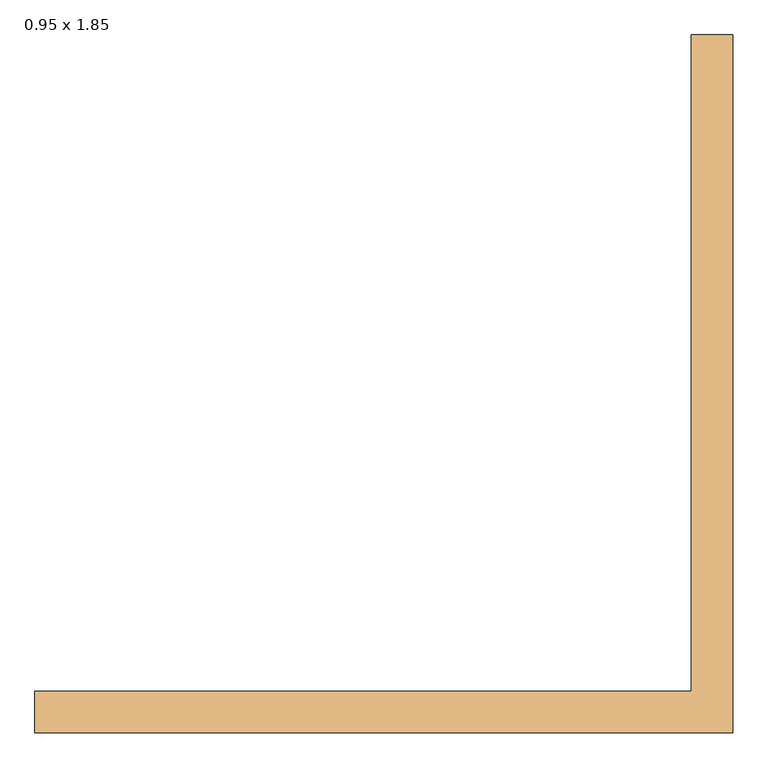
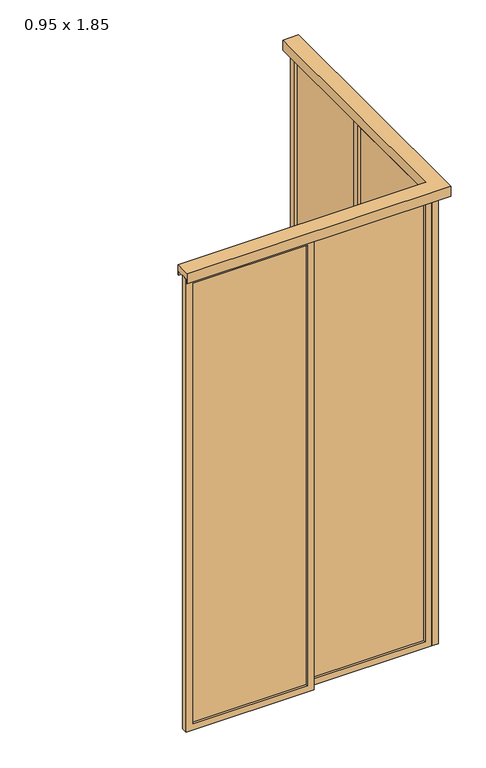
"""IFC4 building model written with IfcOpenShell, lengths in millimetres: door geometry, CC_ND-200_BOX-L-BANHEIRO : 0.95 x 1.85."""

import ifcopenshell
import ifcopenshell.guid

model = None  # the IFC model being written
_history = None  # IfcOwnerHistory: only IFC2X3 demands one
_inside = {}  # id of a spatial element -> (the spatial element, [elements in it])
_under = {}  # id of a project, library or spatial element -> (it, [spatial elements below it])
_declared = {}  # id of a project -> (the project, [libraries it declares])
_typed = {}  # id of a type object -> (the type object, [elements of that type])
_made_of = {}  # id of a material, layer set ... -> (it, [elements and type objects made of it])


def new_model(schema):
    """Start an empty IFC model of exactly this schema.

    Asked for "IFC4X3", IfcOpenShell would pick the latest addendum, in which some entities
    have other attributes; the version numbers below select the first issue.
    IFC2X3 requires an IfcOwnerHistory on every rooted entity: one is made here for all.
    """
    global model, _history
    if schema == "IFC4X3":
        model = ifcopenshell.file(schema_version=(4, 3, 0, 0))
    else:
        model = ifcopenshell.file(schema=schema)
    _inside.clear()
    _under.clear()
    _declared.clear()
    _typed.clear()
    _made_of.clear()
    _history = None
    if model.schema == "IFC2X3":
        org = make("IfcOrganization", Name="unknown")
        user = make(
            "IfcPersonAndOrganization",
            ThePerson=make("IfcPerson", FamilyName="unknown"),
            TheOrganization=org,
        )
        app = make(
            "IfcApplication",
            ApplicationDeveloper=org,
            Version="unknown",
            ApplicationFullName="unknown",
            ApplicationIdentifier="unknown",
        )
        _history = make(
            "IfcOwnerHistory",
            OwningUser=user,
            OwningApplication=app,
            ChangeAction="ADDED",
            CreationDate=0,
        )
    return model


def make(cls, **values):
    """One entity of the class cls with the attributes given. An attribute that is None is left unset."""
    return model.create_entity(
        cls, **{name: value for name, value in values.items() if value is not None}
    )


def rooted(cls, **values):
    """An entity with a GlobalId (a new one), such as an element, a storey or a relation."""
    return make(cls, GlobalId=ifcopenshell.guid.new(), OwnerHistory=_history, **values)


def si_unit(unit_type, name, prefix=None):
    """IfcSIUnit, for example si_unit("LENGTHUNIT", "METRE", prefix="MILLI")."""
    return make("IfcSIUnit", UnitType=unit_type, Prefix=prefix, Name=name)


def assignment(units):
    """IfcUnitAssignment: the units of a project."""
    return None if units is None else make("IfcUnitAssignment", Units=units)


def point(xyz):
    """IfcCartesianPoint."""
    return None if xyz is None else make("IfcCartesianPoint", Coordinates=xyz)


def direction(xyz):
    """IfcDirection."""
    return None if xyz is None else make("IfcDirection", DirectionRatios=xyz)


def frame(location, z_axis=None, x_axis=None):
    """IfcAxis2Placement3D, a coordinate frame: its origin and axes. An axis left out is left unset."""
    return make(
        "IfcAxis2Placement3D",
        Location=point(location),
        Axis=direction(z_axis),
        RefDirection=direction(x_axis),
    )


def origin():
    """The frame at (0, 0, 0) with its axes left unset."""
    return frame((0.0, 0.0, 0.0))


def origin_with_axes():
    """The frame at (0, 0, 0) with the z axis (0, 0, 1) and the x axis (1, 0, 0) written out."""
    return frame((0.0, 0.0, 0.0), z_axis=(0.0, 0.0, 1.0), x_axis=(1.0, 0.0, 0.0))


def place(relative_to, where):
    """IfcLocalPlacement: puts the frame where relative to a parent placement (None: the world)."""
    return make(
        "IfcLocalPlacement", PlacementRelTo=relative_to, RelativePlacement=where
    )


def context(
    kind, dimensions, precision=None, world=None, true_north=None, identifier=None
):
    """IfcGeometricRepresentationContext, for example the 3D "Model" context."""
    return make(
        "IfcGeometricRepresentationContext",
        ContextIdentifier=identifier,
        ContextType=kind,
        CoordinateSpaceDimension=dimensions,
        Precision=precision,
        WorldCoordinateSystem=world,
        TrueNorth=true_north,
    )


def project(units=None, contexts=None):
    """IfcProject with its units and contexts."""
    return rooted(
        "IfcProject",
        Name="project",
        RepresentationContexts=contexts,
        UnitsInContext=assignment(units),
    )


def spatial(cls, under=None, at=None, **own):
    """A site, building, storey or space (cls), placed at a placement, below another one or the project."""
    s = rooted(cls, ObjectPlacement=at, **own)
    if under is not None:
        _under.setdefault(under.id(), (under, []))[1].append(s)
    return s


def polyline(points):
    """IfcPolyline through the points."""
    return make("IfcPolyline", Points=[point(p) for p in points])


def outline(outer, holes=None, kind="AREA"):
    """IfcArbitraryClosedProfileDef: a profile drawn as a closed curve; with holes, ...WithVoids."""
    if holes is None:
        return make("IfcArbitraryClosedProfileDef", ProfileType=kind, OuterCurve=outer)
    return make(
        "IfcArbitraryProfileDefWithVoids",
        ProfileType=kind,
        OuterCurve=outer,
        InnerCurves=holes,
    )


def extrude(swept, where, along, depth):
    """IfcExtrudedAreaSolid: the profile swept, set in the frame where, extruded along a direction by depth."""
    return make(
        "IfcExtrudedAreaSolid",
        SweptArea=swept,
        Position=where,
        ExtrudedDirection=direction(along),
        Depth=depth,
    )


def faces_of(points, faces, orient=None, outer=None):
    """IfcFace entities. A face is a list of loops; a loop is a list of indices into points, from 0.

    orient and outer hold one flag for each loop. By default every Orientation is true, the
    first loop of a face is its IfcFaceOuterBound and the others are IfcFaceBound.
    """
    made = []
    for i, loops in enumerate(faces):
        bounds = []
        for j, loop in enumerate(loops):
            is_outer = j == 0 if outer is None else outer[i][j]
            bounds.append(
                make(
                    "IfcFaceOuterBound" if is_outer else "IfcFaceBound",
                    Bound=make("IfcPolyLoop", Polygon=[points[k] for k in loop]),
                    Orientation=True if orient is None else orient[i][j],
                )
            )
        made.append(make("IfcFace", Bounds=bounds))
    return made


def faceted_brep(points, faces, orient=None, outer=None, voids=None):
    """IfcFacetedBrep: a solid bounded by flat faces; with voids (closed shells), ...WithVoids."""
    shared = [point(p) for p in points]
    hull = make("IfcClosedShell", CfsFaces=faces_of(shared, faces, orient, outer))
    if voids is None:
        return make("IfcFacetedBrep", Outer=hull)
    return make(
        "IfcFacetedBrepWithVoids",
        Outer=hull,
        Voids=[
            make(cls, CfsFaces=faces_of(shared, fs, o, b)) for cls, fs, o, b in voids
        ],
    )


def shape(context_of_items, identifier, shape_type, items):
    """IfcShapeRepresentation: the items that make up one representation, for example the "Body"."""
    return make(
        "IfcShapeRepresentation",
        ContextOfItems=context_of_items,
        RepresentationIdentifier=identifier,
        RepresentationType=shape_type,
        Items=items,
    )


def source(mapping_origin, context_of_items, identifier, shape_type, items):
    """IfcRepresentationMap: a shape defined once, which mapped items show again and again."""
    return make(
        "IfcRepresentationMap",
        MappingOrigin=mapping_origin,
        MappedRepresentation=shape(context_of_items, identifier, shape_type, items),
    )


def transform(
    local_origin,
    x_axis=None,
    y_axis=None,
    z_axis=None,
    scale=None,
    scale2=None,
    scale3=None,
    uniform=True,
):
    """IfcCartesianTransformationOperator3D, or its non-uniform kind. x_axis, y_axis, z_axis: its Axis1, 2, 3."""
    if uniform:
        return make(
            "IfcCartesianTransformationOperator3D",
            Axis1=direction(x_axis),
            Axis2=direction(y_axis),
            LocalOrigin=point(local_origin),
            Scale=scale,
            Axis3=direction(z_axis),
        )
    return make(
        "IfcCartesianTransformationOperator3DnonUniform",
        Axis1=direction(x_axis),
        Axis2=direction(y_axis),
        LocalOrigin=point(local_origin),
        Scale=scale,
        Axis3=direction(z_axis),
        Scale2=scale2,
        Scale3=scale3,
    )


def mapped(mapping_source, mapping_target):
    """IfcMappedItem: shows the shape of a source again, moved by a transform."""
    return make(
        "IfcMappedItem", MappingSource=mapping_source, MappingTarget=mapping_target
    )


def made_of(thing, what):
    """Note that an element or type object is made of a material, layer set ...; save() writes the relation."""
    if what is not None:
        _made_of.setdefault(what.id(), (what, []))[1].append(thing)
    return thing


def element(
    cls,
    number,
    at=None,
    inside=None,
    cuts=None,
    type_object=None,
    material=None,
    context=None,
    identifier="Body",
    shape_type=None,
    held_by="IfcProductDefinitionShape",
    body=None,
    shapes=None,
    **own,
):
    """One element of the class cls, such as IfcWall. Its Tag is "e" and its number.

    at: its placement. inside: the storey or other place that contains it. cuts: it is an
    opening in that element (IfcRelVoidsElement). A single representation is given by context,
    identifier, shape_type and body (its items); several are given by shapes. held_by: the class
    of the entity that holds the representations. save() writes the other relations.
    """
    e = rooted(cls, Tag="e%d" % number, ObjectPlacement=at, **own)
    if body is not None:
        shapes = [shape(context, identifier, shape_type, body)]
    if shapes is not None:
        e.Representation = make(held_by, Representations=shapes)
    if inside is not None:
        _inside.setdefault(inside.id(), (inside, []))[1].append(e)
    if cuts is not None:
        rooted(
            "IfcRelVoidsElement", RelatingBuildingElement=cuts, RelatedOpeningElement=e
        )
    if type_object is not None:
        _typed.setdefault(type_object.id(), (type_object, []))[1].append(e)
    return made_of(e, material)


def aggregate(whole, parts):
    """IfcRelAggregates: a whole, such as a stair, and the parts it consists of."""
    return rooted("IfcRelAggregates", RelatingObject=whole, RelatedObjects=parts)


def save(model, path):
    """Write the relations noted so far, then the file.

    IfcRelAggregates (storeys below a building ...), IfcRelContainedInSpatialStructure (elements
    in a storey), IfcRelDefinesByType, IfcRelAssociatesMaterial and IfcRelDeclares: one each for
    every whole, place, type object, material and project.
    """
    for whole, parts in _under.values():
        aggregate(whole, parts)
    for where, things in _inside.values():
        rooted(
            "IfcRelContainedInSpatialStructure",
            RelatedElements=things,
            RelatingStructure=where,
        )
    for kind, things in _typed.values():
        rooted("IfcRelDefinesByType", RelatedObjects=things, RelatingType=kind)
    for what, things in _made_of.values():
        rooted("IfcRelAssociatesMaterial", RelatedObjects=things, RelatingMaterial=what)
    for by, libraries in _declared.values():
        rooted("IfcRelDeclares", RelatingContext=by, RelatedDefinitions=libraries)
    model.write(path)


def door_0_95_x_1_85_64086e03(model_context):
    return source(origin(), model_context, "Body", "SolidModel", [
        extrude(outline(polyline([(975.0, 50.0), (975.0, 25.0), (950.0, 25.0), (950.0, 50.0), (975.0, 50.0)])), origin_with_axes(), (0.0, 0.0, 1.0), 1825.0),
        extrude(outline(polyline([(965.0, 527.5), (965.0, 60.0), (960.0, 60.0), (960.0, 527.5), (965.0, 527.5)])), frame((0.0, 0.0, 10.0), z_axis=(0.0, 0.0, 1.0), x_axis=(1.0, 0.0, 0.0)), (0.0, 0.0, 1.0), 1805.0),
        faceted_brep([(975.0, 512.5, 1800.0), (965.0, 512.5, 1800.0), (965.0, 512.5, 25.0), (975.0, 512.5, 25.0), (965.0, 527.5, 1815.0), (965.0, 527.5, 10.0), (965.0, 60.0, 10.0), (965.0, 60.0, 1815.0), (965.0, 75.0, 1800.0), (965.0, 75.0, 25.0), (975.0, 75.0, 25.0), (975.0, 50.0, 1825.0), (975.0, 50.0, 0.0), (975.0, 537.5, 0.0), (975.0, 537.5, 1825.0), (975.0, 75.0, 1800.0), (950.0, 537.5, 1825.0), (950.0, 537.5, 0.0), (950.0, 50.0, 0.0), (950.0, 50.0, 1825.0), (950.0, 75.0, 1800.0), (950.0, 75.0, 25.0), (950.0, 512.5, 25.0), (950.0, 512.5, 1800.0), (960.0, 75.0, 25.0), (960.0, 75.0, 1800.0), (960.0, 512.5, 25.0), (960.0, 512.5, 1800.0), (960.0, 527.5, 1815.0), (960.0, 527.5, 10.0), (960.0, 60.0, 1815.0), (960.0, 60.0, 10.0)], [[[0, 1, 2, 3]], [[4, 5, 6, 7], [8, 9, 2, 1]], [[3, 2, 9, 10]], [[11, 12, 13, 14], [0, 3, 10, 15]], [[16, 14, 13, 17]], [[17, 13, 12, 18]], [[16, 17, 18, 19], [20, 21, 22, 23]], [[10, 9, 8, 15]], [[18, 12, 11, 19]], [[24, 21, 20, 25]], [[26, 22, 21, 24]], [[27, 23, 22, 26]], [[4, 28, 29, 5]], [[30, 31, 29, 28], [27, 26, 24, 25]], [[5, 29, 31, 6]], [[6, 31, 30, 7]], [[15, 8, 1, 0]], [[19, 11, 14, 16]], [[7, 30, 28, 4]], [[25, 20, 23, 27]]]),
        extrude(outline(polyline([(990.0, 990.0), (990.0, 522.5), (985.0, 522.5), (985.0, 990.0), (990.0, 990.0)])), frame((0.0, 0.0, 10.0), z_axis=(0.0, 0.0, 1.0), x_axis=(1.0, 0.0, 0.0)), (0.0, 0.0, 1.0), 1805.0),
        faceted_brep([(1000.0, 975.0, 1800.0), (990.0, 975.0, 1800.0), (990.0, 975.0, 25.0), (1000.0, 975.0, 25.0), (990.0, 990.0, 1815.0), (990.0, 990.0, 10.0), (990.0, 522.5, 10.0), (990.0, 522.5, 1815.0), (990.0, 537.5, 1800.0), (990.0, 537.5, 25.0), (1000.0, 537.5, 25.0), (1000.0, 512.5, 1825.0), (1000.0, 512.5, 0.0), (1000.0, 1000.0, 0.0), (1000.0, 1000.0, 1825.0), (1000.0, 537.5, 1800.0), (975.0, 1000.0, 1825.0), (975.0, 1000.0, 0.0), (975.0, 512.5, 0.0), (975.0, 512.5, 1825.0), (975.0, 537.5, 1800.0), (975.0, 537.5, 25.0), (975.0, 975.0, 25.0), (975.0, 975.0, 1800.0), (985.0, 537.5, 25.0), (985.0, 537.5, 1800.0), (985.0, 975.0, 25.0), (985.0, 975.0, 1800.0), (985.0, 990.0, 1815.0), (985.0, 990.0, 10.0), (985.0, 522.5, 1815.0), (985.0, 522.5, 10.0)], [[[0, 1, 2, 3]], [[4, 5, 6, 7], [8, 9, 2, 1]], [[3, 2, 9, 10]], [[11, 12, 13, 14], [0, 3, 10, 15]], [[16, 14, 13, 17]], [[17, 13, 12, 18]], [[16, 17, 18, 19], [20, 21, 22, 23]], [[10, 9, 8, 15]], [[18, 12, 11, 19]], [[24, 21, 20, 25]], [[26, 22, 21, 24]], [[27, 23, 22, 26]], [[4, 28, 29, 5]], [[30, 31, 29, 28], [27, 26, 24, 25]], [[5, 29, 31, 6]], [[6, 31, 30, 7]], [[15, 8, 1, 0]], [[19, 11, 14, 16]], [[7, 30, 28, 4]], [[25, 20, 23, 27]]]),
        extrude(outline(polyline([(477.5, 15.0), (477.5, 10.0), (10.0, 10.0), (10.0, 15.0), (477.5, 15.0)])), frame((0.0, 0.0, 10.0), z_axis=(0.0, 0.0, 1.0), x_axis=(1.0, 0.0, 0.0)), (0.0, 0.0, 1.0), 1805.0),
        faceted_brep([(462.5, 15.0, 1800.0), (462.5, 25.0, 1800.0), (462.5, 25.0, 25.0), (462.5, 15.0, 25.0), (487.5, 25.0, 1825.0), (487.5, 25.0, 0.0), (0.0, 25.0, 0.0), (0.0, 25.0, 1825.0), (25.0, 25.0, 1800.0), (25.0, 25.0, 25.0), (25.0, 15.0, 25.0), (10.0, 15.0, 1815.0), (10.0, 15.0, 10.0), (477.5, 15.0, 10.0), (477.5, 15.0, 1815.0), (25.0, 15.0, 1800.0), (487.5, 0.0, 1825.0), (487.5, 0.0, 0.0), (0.0, 0.0, 1825.0), (0.0, 0.0, 0.0), (462.5, 0.0, 1800.0), (462.5, 0.0, 25.0), (25.0, 0.0, 25.0), (25.0, 0.0, 1800.0), (462.5, 10.0, 1800.0), (462.5, 10.0, 25.0), (25.0, 10.0, 25.0), (25.0, 10.0, 1800.0), (477.5, 10.0, 1815.0), (477.5, 10.0, 10.0), (10.0, 10.0, 10.0), (10.0, 10.0, 1815.0)], [[[0, 1, 2, 3]], [[4, 5, 6, 7], [8, 9, 2, 1]], [[3, 2, 9, 10]], [[11, 12, 13, 14], [0, 3, 10, 15]], [[4, 16, 17, 5]], [[18, 19, 17, 16], [20, 21, 22, 23]], [[5, 17, 19, 6]], [[10, 9, 8, 15]], [[6, 19, 18, 7]], [[20, 24, 25, 21]], [[21, 25, 26, 22]], [[22, 26, 27, 23]], [[28, 14, 13, 29]], [[29, 13, 12, 30]], [[28, 29, 30, 31], [27, 26, 25, 24]], [[30, 12, 11, 31]], [[15, 8, 1, 0]], [[7, 18, 16, 4]], [[31, 11, 14, 28]], [[23, 27, 24, 20]]]),
        extrude(outline(polyline([(940.0, 40.0), (940.0, 35.0), (472.5, 35.0), (472.5, 40.0), (940.0, 40.0)])), frame((0.0, 0.0, 10.0), z_axis=(0.0, 0.0, 1.0), x_axis=(1.0, 0.0, 0.0)), (0.0, 0.0, 1.0), 1805.0),
        faceted_brep([(925.0, 40.0, 1800.0), (925.0, 50.0, 1800.0), (925.0, 50.0, 25.0), (925.0, 40.0, 25.0), (950.0, 50.0, 1825.0), (950.0, 50.0, 0.0), (462.5, 50.0, 0.0), (462.5, 50.0, 1825.0), (487.5, 50.0, 1800.0), (487.5, 50.0, 25.0), (487.5, 40.0, 25.0), (472.5, 40.0, 1815.0), (472.5, 40.0, 10.0), (940.0, 40.0, 10.0), (940.0, 40.0, 1815.0), (487.5, 40.0, 1800.0), (950.0, 25.0, 1825.0), (950.0, 25.0, 0.0), (462.5, 25.0, 1825.0), (462.5, 25.0, 0.0), (925.0, 25.0, 1800.0), (925.0, 25.0, 25.0), (487.5, 25.0, 25.0), (487.5, 25.0, 1800.0), (925.0, 35.0, 1800.0), (925.0, 35.0, 25.0), (487.5, 35.0, 25.0), (487.5, 35.0, 1800.0), (940.0, 35.0, 1815.0), (940.0, 35.0, 10.0), (472.5, 35.0, 10.0), (472.5, 35.0, 1815.0)], [[[0, 1, 2, 3]], [[4, 5, 6, 7], [8, 9, 2, 1]], [[3, 2, 9, 10]], [[11, 12, 13, 14], [0, 3, 10, 15]], [[4, 16, 17, 5]], [[18, 19, 17, 16], [20, 21, 22, 23]], [[5, 17, 19, 6]], [[10, 9, 8, 15]], [[6, 19, 18, 7]], [[20, 24, 25, 21]], [[21, 25, 26, 22]], [[22, 26, 27, 23]], [[28, 14, 13, 29]], [[29, 13, 12, 30]], [[28, 29, 30, 31], [27, 26, 25, 24]], [[30, 12, 11, 31]], [[15, 8, 1, 0]], [[7, 18, 16, 4]], [[31, 11, 14, 28]], [[23, 27, 24, 20]]]),
        faceted_brep([(0.0, -5.0, 1810.0), (0.0, -5.0, 1850.0), (0.0, 55.0, 1850.0), (0.0, 55.0, 1810.0), (0.0, 50.0, 1810.0), (0.0, 50.0, 1825.0), (0.0, 0.0, 1825.0), (0.0, 0.0, 1810.0), (1005.0, 1000.0, 1810.0), (1000.0, 1000.0, 1810.0), (1000.0, 1000.0, 1825.0), (950.0, 1000.0, 1825.0), (950.0, 1000.0, 1810.0), (945.0, 1000.0, 1810.0), (945.0, 1000.0, 1850.0), (1005.0, 1000.0, 1850.0), (1005.0, -5.0, 1810.0), (1005.0, -5.0, 1850.0), (945.0, 55.0, 1850.0), (945.0, 55.0, 1810.0), (950.0, 50.0, 1810.0), (950.0, 50.0, 1825.0), (1000.0, 0.0, 1825.0), (1000.0, 0.0, 1810.0)], [[[0, 1, 2, 3, 4, 5, 6, 7]], [[8, 9, 10, 11, 12, 13, 14, 15]], [[1, 0, 16, 17]], [[2, 1, 17, 15, 14, 18]], [[3, 2, 18, 19]], [[4, 3, 19, 13, 12, 20]], [[5, 4, 20, 21]], [[6, 5, 21, 11, 10, 22]], [[7, 6, 22, 23]], [[0, 7, 23, 9, 8, 16]], [[17, 16, 8, 15]], [[19, 18, 14, 13]], [[21, 20, 12, 11]], [[23, 22, 10, 9]]]),
    ])


if __name__ == "__main__":
    model = new_model("IFC4")
    model_context = context("Model", 3, world=origin())
    ifc_project = project(units=[si_unit("LENGTHUNIT", "METRE", prefix="MILLI")], contexts=[model_context])
    site = spatial("IfcSite", under=ifc_project)
    building = spatial("IfcBuilding", under=site)
    placement = place(None, origin())
    door_0_95_x_1_85_shape = door_0_95_x_1_85_64086e03(model_context)
    element("IfcDoor", 1, ObjectType="CC_ND-200_BOX-L-BANHEIRO : 0.95 x 1.85", at=placement, inside=building, context=model_context, shape_type="MappedRepresentation", body=[
        mapped(door_0_95_x_1_85_shape, transform((0.0, 0.0, 0.0), x_axis=(1.0, 0.0, 0.0), y_axis=(0.0, 1.0, 0.0), z_axis=(0.0, 0.0, 1.0))),
    ])
    save(model, "model.ifc")

# Revit data of these elements
# Type "CC_ND-200_BOX-L-BANHEIRO : 0.95 x 1.85"
#   Type Mark = "144"
#   Width = 0.95 m
#   Material montante = Aluminio
#   Materia vidro = Vidro
# Element 1 (IfcDoor, "CC_ND-200_BOX-L-BANHEIRO : 0.95 x 1.85")
#   Materials on its faces: "Aluminio", "Vidro"
# Materials
#   "Aluminio": class "Genérico", colour RGB 120 120 120, transparency 0, Cost = 0
#   "Vidro": class "Vidro", colour RGB 230 230 230, transparency 0.75, Description = "JANELA COM 04 FOLHAS DE CORRER E VIDRO TRANSPARENTE 6mm", Cost = 0
